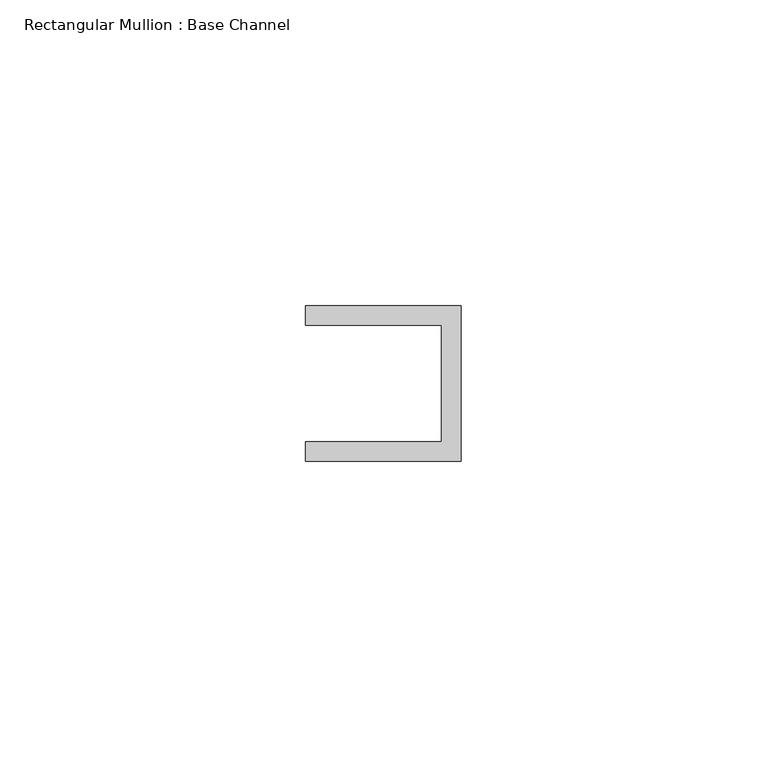
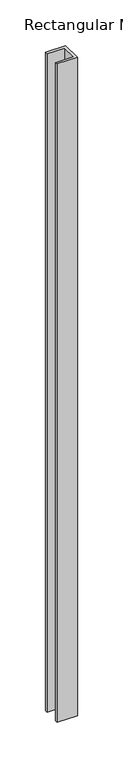
"""IFC4 building model written with IfcOpenShell, lengths in millimetres: member geometry, Rectangular Mullion : Base Channel."""

from ifc_helpers import new_model, si_unit, frame, origin, place, context, project, spatial, polyline, outline, extrude, source, transform, mapped, element, save


def rectangular_mullion_base_channel_1a1b2a0c(model_context):
    return source(origin(), model_context, "Body", "SweptSolid", [
        extrude(outline(polyline([(0.0, 12.7), (0.0, -12.7), (-25.4, -12.7), (-25.4, -9.525), (-3.175, -9.525), (-3.175, 9.525), (-25.4, 9.525), (-25.4, 12.7), (0.0, 12.7)])), frame((0.0, 0.0, -877.8875), z_axis=(0.0, 0.0, 1.0), x_axis=(1.0, 0.0, 0.0)), (0.0, 0.0, 1.0), 877.8875),
    ])


if __name__ == "__main__":
    model = new_model("IFC4")
    model_context = context("Model", 3, world=origin())
    ifc_project = project(units=[si_unit("LENGTHUNIT", "METRE", prefix="MILLI")], contexts=[model_context])
    site = spatial("IfcSite", under=ifc_project)
    building = spatial("IfcBuilding", under=site)
    placement = place(None, origin())
    rectangular_mullion_base_channel_shape = rectangular_mullion_base_channel_1a1b2a0c(model_context)
    element("IfcMember", 1, ObjectType="Rectangular Mullion : Base Channel", at=placement, inside=building, context=model_context, shape_type="MappedRepresentation", body=[
        mapped(rectangular_mullion_base_channel_shape, transform((0.0, 0.0, 0.0), x_axis=(1.0, 0.0, 0.0), y_axis=(0.0, 1.0, 0.0), z_axis=(0.0, 0.0, 1.0))),
    ])
    save(model, "model.ifc")

# Revit data of these elements
# Type "Rectangular Mullion : Base Channel"
#   built-in parameter 1007322 = 0.0833333 (stored number, unit not read)
#   built-in parameter 1007321 = 0.0416667 (stored number, unit not read)
#   built-in parameter 1007320 = -0.03125 (stored number, unit not read)
# Element 1 (IfcMember, "Rectangular Mullion : Base Channel")
#   Materials on its faces: "ALUM"
# Materials
#   "ALUM": class "Generic", colour RGB 157 157 157, transparency 0, Cost = 0
